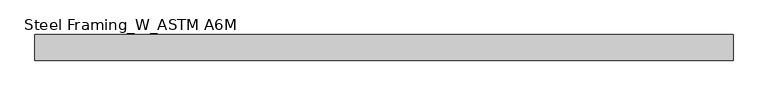
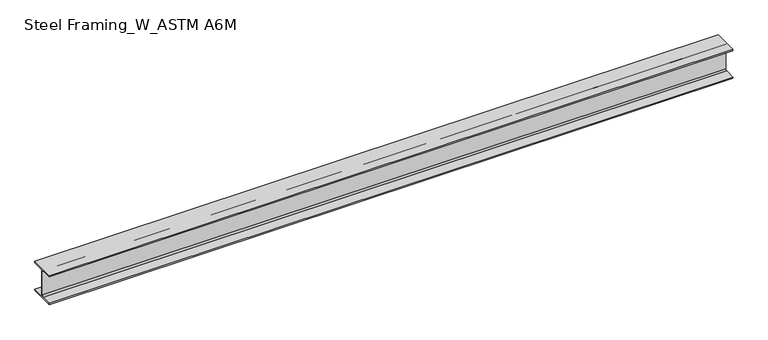
"""IFC4 building model written with IfcOpenShell, lengths in millimetres: beam geometry, Steel Framing_W_ASTM A6M : H_SB_AR_S02_W250x49.1_G5."""

from ifc_helpers import new_model, si_unit, point, frame, frame_2d, origin, place, context, project, spatial, polyline, circle_curve, trimmed, segment, composite_curve, outline, extrude, source, transform, mapped, element, save


def steel_framing_w_astm_a6m_5be407e6(model_context):
    return source(origin(), model_context, "Body", "SweptSolid", [
        extrude(outline(composite_curve([segment(polyline([(101.0, -112.5), (101.0, -123.5), (-101.0, -123.5), (-101.0, -112.5), (-16.385, -112.5)]), True, "CONTINUOUS"), segment(trimmed(circle_curve(frame_2d((-16.385, -99.8)), 12.7), [point((-16.385, -112.5))], [point((-3.685, -99.8))], True, "CARTESIAN"), True, "CONTINUOUS"), segment(polyline([(-3.685, -99.8), (-3.685, 99.8)]), True, "CONTINUOUS"), segment(trimmed(circle_curve(frame_2d((-16.385, 99.8)), 12.7), [point((-3.685, 99.8))], [point((-16.385, 112.5))], True, "CARTESIAN"), True, "CONTINUOUS"), segment(polyline([(-16.385, 112.5), (-101.0, 112.5), (-101.0, 123.5), (101.0, 123.5), (101.0, 112.5), (16.385, 112.5)]), True, "CONTINUOUS"), segment(trimmed(circle_curve(frame_2d((16.385, 99.8)), 12.7), [point((16.385, 112.5))], [point((3.685, 99.8))], True, "CARTESIAN"), True, "CONTINUOUS"), segment(polyline([(3.685, 99.8), (3.685, -99.8)]), True, "CONTINUOUS"), segment(trimmed(circle_curve(frame_2d((16.385, -99.8)), 12.7), [point((3.685, -99.8))], [point((16.385, -112.5))], True, "CARTESIAN"), True, "CONTINUOUS"), segment(polyline([(16.385, -112.5), (101.0, -112.5)]), True, "CONTINUOUS")], self_intersect=False)), frame((-2753.8, 0.0, 0.0), z_axis=(1.0, 0.0, 0.0), x_axis=(0.0, 1.0, 0.0)), (0.0, 0.0, 1.0), 5507.6),
    ])


if __name__ == "__main__":
    model = new_model("IFC4")
    model_context = context("Model", 3, world=origin())
    ifc_project = project(units=[si_unit("LENGTHUNIT", "METRE", prefix="MILLI")], contexts=[model_context])
    site = spatial("IfcSite", under=ifc_project)
    building = spatial("IfcBuilding", under=site)
    placement = place(None, origin())
    steel_framing_w_astm_a6m_shape = steel_framing_w_astm_a6m_5be407e6(model_context)
    element("IfcBeam", 1, ObjectType="Steel Framing_W_ASTM A6M : H_SB_AR_S02_W250x49.1_G5", at=placement, inside=building, context=model_context, shape_type="MappedRepresentation", body=[
        mapped(steel_framing_w_astm_a6m_shape, transform((0.0, 0.0, 0.0), x_axis=(1.0, 0.0, 0.0), y_axis=(0.0, 1.0, 0.0), z_axis=(0.0, 0.0, 1.0))),
    ])
    save(model, "model.ifc")

# Revit data of these elements
# Type "Steel Framing_W_ASTM A6M : H_SB_AR_S02_W250x49.1_G5"
#   Type Mark = "G5"
#   Section Name Key = "W10x33"
#   Width = 20.2 cm
#   Web Thickness = 0.737 cm
#   Web Fillet = 1.27 cm
#   Warping Constant = 212000.0 cm⁶
#   Torsional Moment of Inertia = 24.30 cm⁴
#   Section Area = 62.6 cm²
#   Plastic Modulus weak axis = 229.0 cm³
#   Plastic Modulus strong axis = 636.0 cm³
#   Perimeter = 1.27 m²/m
#   Nominal Weight = 49.10 kgf/m
#   Moment of Inertia weak axis = 1520.00 cm⁴
#   Moment of Inertia strong axis = 7120.00 cm⁴
#   Height = 24.7 cm
#   Flange Thickness = 1.1 cm
#   Elastic Modulus weak axis = 151.0 cm³
#   Elastic Modulus strong axis = 574.0 cm³
#   Centroid Vertical = 12.35 cm
#   Centroid Horizontal = 10.1 cm
#   Length [instance default] = 1500 mm
#   Structural Material [instance default] = Steel, 45-345
#   Bolt Spacing = 0
#   Assembly Code = ""
# Element 1 (IfcBeam, "Steel Framing_W_ASTM A6M : H_SB_AR_S02_W250x49.1_G5")
#   Materials on its faces: "Steel, 45-345"
# Materials
#   "Steel, 45-345": class "Metal", colour RGB 189 187 185, transparency 0, Description = "Steel 345 MPa", Cost = 0
